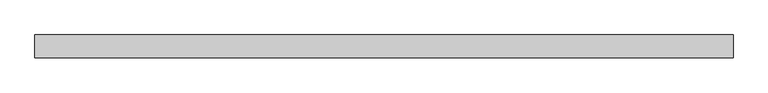
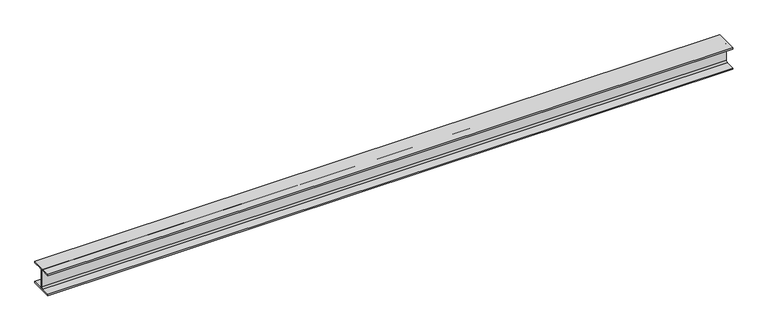
"""IFC4 building model written with IfcOpenShell, lengths in millimetres: beam geometry, 0912_Steel Framing_H-KSD3502 : H_SB_ASB_H-200x200x8x12."""

import ifcopenshell
import ifcopenshell.guid

model = None  # the IFC model being written
_history = None  # IfcOwnerHistory: only IFC2X3 demands one
_inside = {}  # id of a spatial element -> (the spatial element, [elements in it])
_under = {}  # id of a project, library or spatial element -> (it, [spatial elements below it])
_declared = {}  # id of a project -> (the project, [libraries it declares])
_typed = {}  # id of a type object -> (the type object, [elements of that type])
_made_of = {}  # id of a material, layer set ... -> (it, [elements and type objects made of it])


def new_model(schema):
    """Start an empty IFC model of exactly this schema.

    Asked for "IFC4X3", IfcOpenShell would pick the latest addendum, in which some entities
    have other attributes; the version numbers below select the first issue.
    IFC2X3 requires an IfcOwnerHistory on every rooted entity: one is made here for all.
    """
    global model, _history
    if schema == "IFC4X3":
        model = ifcopenshell.file(schema_version=(4, 3, 0, 0))
    else:
        model = ifcopenshell.file(schema=schema)
    _inside.clear()
    _under.clear()
    _declared.clear()
    _typed.clear()
    _made_of.clear()
    _history = None
    if model.schema == "IFC2X3":
        org = make("IfcOrganization", Name="unknown")
        user = make(
            "IfcPersonAndOrganization",
            ThePerson=make("IfcPerson", FamilyName="unknown"),
            TheOrganization=org,
        )
        app = make(
            "IfcApplication",
            ApplicationDeveloper=org,
            Version="unknown",
            ApplicationFullName="unknown",
            ApplicationIdentifier="unknown",
        )
        _history = make(
            "IfcOwnerHistory",
            OwningUser=user,
            OwningApplication=app,
            ChangeAction="ADDED",
            CreationDate=0,
        )
    return model


def make(cls, **values):
    """One entity of the class cls with the attributes given. An attribute that is None is left unset."""
    return model.create_entity(
        cls, **{name: value for name, value in values.items() if value is not None}
    )


def rooted(cls, **values):
    """An entity with a GlobalId (a new one), such as an element, a storey or a relation."""
    return make(cls, GlobalId=ifcopenshell.guid.new(), OwnerHistory=_history, **values)


def si_unit(unit_type, name, prefix=None):
    """IfcSIUnit, for example si_unit("LENGTHUNIT", "METRE", prefix="MILLI")."""
    return make("IfcSIUnit", UnitType=unit_type, Prefix=prefix, Name=name)


def assignment(units):
    """IfcUnitAssignment: the units of a project."""
    return None if units is None else make("IfcUnitAssignment", Units=units)


def point(xyz):
    """IfcCartesianPoint."""
    return None if xyz is None else make("IfcCartesianPoint", Coordinates=xyz)


def direction(xyz):
    """IfcDirection."""
    return None if xyz is None else make("IfcDirection", DirectionRatios=xyz)


def frame(location, z_axis=None, x_axis=None):
    """IfcAxis2Placement3D, a coordinate frame: its origin and axes. An axis left out is left unset."""
    return make(
        "IfcAxis2Placement3D",
        Location=point(location),
        Axis=direction(z_axis),
        RefDirection=direction(x_axis),
    )


def frame_2d(location, x_axis=None):
    """IfcAxis2Placement2D, a coordinate frame in the plane: its origin and x axis."""
    return make(
        "IfcAxis2Placement2D", Location=point(location), RefDirection=direction(x_axis)
    )


def origin():
    """The frame at (0, 0, 0) with its axes left unset."""
    return frame((0.0, 0.0, 0.0))


def place(relative_to, where):
    """IfcLocalPlacement: puts the frame where relative to a parent placement (None: the world)."""
    return make(
        "IfcLocalPlacement", PlacementRelTo=relative_to, RelativePlacement=where
    )


def context(
    kind, dimensions, precision=None, world=None, true_north=None, identifier=None
):
    """IfcGeometricRepresentationContext, for example the 3D "Model" context."""
    return make(
        "IfcGeometricRepresentationContext",
        ContextIdentifier=identifier,
        ContextType=kind,
        CoordinateSpaceDimension=dimensions,
        Precision=precision,
        WorldCoordinateSystem=world,
        TrueNorth=true_north,
    )


def project(units=None, contexts=None):
    """IfcProject with its units and contexts."""
    return rooted(
        "IfcProject",
        Name="project",
        RepresentationContexts=contexts,
        UnitsInContext=assignment(units),
    )


def spatial(cls, under=None, at=None, **own):
    """A site, building, storey or space (cls), placed at a placement, below another one or the project."""
    s = rooted(cls, ObjectPlacement=at, **own)
    if under is not None:
        _under.setdefault(under.id(), (under, []))[1].append(s)
    return s


def polyline(points):
    """IfcPolyline through the points."""
    return make("IfcPolyline", Points=[point(p) for p in points])


def circle_curve(where, radius):
    """IfcCircle in the frame where."""
    return make("IfcCircle", Position=where, Radius=radius)


def trimmed(basis, trim1, trim2, sense, master):
    """IfcTrimmedCurve: the piece of a basis curve between two trims."""
    return make(
        "IfcTrimmedCurve",
        BasisCurve=basis,
        Trim1=trim1,
        Trim2=trim2,
        SenseAgreement=sense,
        MasterRepresentation=master,
    )


def segment(curve, same_sense, transition):
    """IfcCompositeCurveSegment."""
    return make(
        "IfcCompositeCurveSegment",
        Transition=transition,
        SameSense=same_sense,
        ParentCurve=curve,
    )


def composite_curve(segments, self_intersect=None):
    """IfcCompositeCurve: segments joined end to end."""
    return make("IfcCompositeCurve", Segments=segments, SelfIntersect=self_intersect)


def outline(outer, holes=None, kind="AREA"):
    """IfcArbitraryClosedProfileDef: a profile drawn as a closed curve; with holes, ...WithVoids."""
    if holes is None:
        return make("IfcArbitraryClosedProfileDef", ProfileType=kind, OuterCurve=outer)
    return make(
        "IfcArbitraryProfileDefWithVoids",
        ProfileType=kind,
        OuterCurve=outer,
        InnerCurves=holes,
    )


def extrude(swept, where, along, depth):
    """IfcExtrudedAreaSolid: the profile swept, set in the frame where, extruded along a direction by depth."""
    return make(
        "IfcExtrudedAreaSolid",
        SweptArea=swept,
        Position=where,
        ExtrudedDirection=direction(along),
        Depth=depth,
    )


def shape(context_of_items, identifier, shape_type, items):
    """IfcShapeRepresentation: the items that make up one representation, for example the "Body"."""
    return make(
        "IfcShapeRepresentation",
        ContextOfItems=context_of_items,
        RepresentationIdentifier=identifier,
        RepresentationType=shape_type,
        Items=items,
    )


def source(mapping_origin, context_of_items, identifier, shape_type, items):
    """IfcRepresentationMap: a shape defined once, which mapped items show again and again."""
    return make(
        "IfcRepresentationMap",
        MappingOrigin=mapping_origin,
        MappedRepresentation=shape(context_of_items, identifier, shape_type, items),
    )


def transform(
    local_origin,
    x_axis=None,
    y_axis=None,
    z_axis=None,
    scale=None,
    scale2=None,
    scale3=None,
    uniform=True,
):
    """IfcCartesianTransformationOperator3D, or its non-uniform kind. x_axis, y_axis, z_axis: its Axis1, 2, 3."""
    if uniform:
        return make(
            "IfcCartesianTransformationOperator3D",
            Axis1=direction(x_axis),
            Axis2=direction(y_axis),
            LocalOrigin=point(local_origin),
            Scale=scale,
            Axis3=direction(z_axis),
        )
    return make(
        "IfcCartesianTransformationOperator3DnonUniform",
        Axis1=direction(x_axis),
        Axis2=direction(y_axis),
        LocalOrigin=point(local_origin),
        Scale=scale,
        Axis3=direction(z_axis),
        Scale2=scale2,
        Scale3=scale3,
    )


def mapped(mapping_source, mapping_target):
    """IfcMappedItem: shows the shape of a source again, moved by a transform."""
    return make(
        "IfcMappedItem", MappingSource=mapping_source, MappingTarget=mapping_target
    )


def made_of(thing, what):
    """Note that an element or type object is made of a material, layer set ...; save() writes the relation."""
    if what is not None:
        _made_of.setdefault(what.id(), (what, []))[1].append(thing)
    return thing


def element(
    cls,
    number,
    at=None,
    inside=None,
    cuts=None,
    type_object=None,
    material=None,
    context=None,
    identifier="Body",
    shape_type=None,
    held_by="IfcProductDefinitionShape",
    body=None,
    shapes=None,
    **own,
):
    """One element of the class cls, such as IfcWall. Its Tag is "e" and its number.

    at: its placement. inside: the storey or other place that contains it. cuts: it is an
    opening in that element (IfcRelVoidsElement). A single representation is given by context,
    identifier, shape_type and body (its items); several are given by shapes. held_by: the class
    of the entity that holds the representations. save() writes the other relations.
    """
    e = rooted(cls, Tag="e%d" % number, ObjectPlacement=at, **own)
    if body is not None:
        shapes = [shape(context, identifier, shape_type, body)]
    if shapes is not None:
        e.Representation = make(held_by, Representations=shapes)
    if inside is not None:
        _inside.setdefault(inside.id(), (inside, []))[1].append(e)
    if cuts is not None:
        rooted(
            "IfcRelVoidsElement", RelatingBuildingElement=cuts, RelatedOpeningElement=e
        )
    if type_object is not None:
        _typed.setdefault(type_object.id(), (type_object, []))[1].append(e)
    return made_of(e, material)


def aggregate(whole, parts):
    """IfcRelAggregates: a whole, such as a stair, and the parts it consists of."""
    return rooted("IfcRelAggregates", RelatingObject=whole, RelatedObjects=parts)


def save(model, path):
    """Write the relations noted so far, then the file.

    IfcRelAggregates (storeys below a building ...), IfcRelContainedInSpatialStructure (elements
    in a storey), IfcRelDefinesByType, IfcRelAssociatesMaterial and IfcRelDeclares: one each for
    every whole, place, type object, material and project.
    """
    for whole, parts in _under.values():
        aggregate(whole, parts)
    for where, things in _inside.values():
        rooted(
            "IfcRelContainedInSpatialStructure",
            RelatedElements=things,
            RelatingStructure=where,
        )
    for kind, things in _typed.values():
        rooted("IfcRelDefinesByType", RelatedObjects=things, RelatingType=kind)
    for what, things in _made_of.values():
        rooted("IfcRelAssociatesMaterial", RelatedObjects=things, RelatingMaterial=what)
    for by, libraries in _declared.values():
        rooted("IfcRelDeclares", RelatingContext=by, RelatedDefinitions=libraries)
    model.write(path)


def beam_026c0679(model_context):
    return source(origin(), model_context, "Body", "SweptSolid", [
        extrude(outline(composite_curve([segment(polyline([(100.0, -88.0), (100.0, -100.0), (-100.0, -100.0), (-100.0, -88.0), (-17.0, -88.0)]), True, "CONTINUOUS"), segment(trimmed(circle_curve(frame_2d((-17.0, -75.0)), 13.0), [point((-17.0, -88.0))], [point((-4.0, -75.0))], True, "CARTESIAN"), True, "CONTINUOUS"), segment(polyline([(-4.0, -75.0), (-4.0, 75.0)]), True, "CONTINUOUS"), segment(trimmed(circle_curve(frame_2d((-17.0, 75.0)), 13.0), [point((-4.0, 75.0))], [point((-17.0, 88.0))], True, "CARTESIAN"), True, "CONTINUOUS"), segment(polyline([(-17.0, 88.0), (-100.0, 88.0), (-100.0, 100.0), (100.0, 100.0), (100.0, 88.0), (17.0, 88.0)]), True, "CONTINUOUS"), segment(trimmed(circle_curve(frame_2d((17.0, 75.0)), 13.0), [point((17.0, 88.0))], [point((4.0, 75.0))], True, "CARTESIAN"), True, "CONTINUOUS"), segment(polyline([(4.0, 75.0), (4.0, -75.0)]), True, "CONTINUOUS"), segment(trimmed(circle_curve(frame_2d((17.0, -75.0)), 13.0), [point((4.0, -75.0))], [point((17.0, -88.0))], True, "CARTESIAN"), True, "CONTINUOUS"), segment(polyline([(17.0, -88.0), (100.0, -88.0)]), True, "CONTINUOUS")], self_intersect=False)), frame((-3041.4802947, 0.0, 0.0), z_axis=(1.0, 0.0, 0.0), x_axis=(0.0, 1.0, 0.0)), (0.0, 0.0, 1.0), 6052.7309213),
    ])


if __name__ == "__main__":
    model = new_model("IFC4")
    model_context = context("Model", 3, world=origin())
    ifc_project = project(units=[si_unit("LENGTHUNIT", "METRE", prefix="MILLI")], contexts=[model_context])
    site = spatial("IfcSite", under=ifc_project)
    building = spatial("IfcBuilding", under=site)
    placement = place(None, origin())
    beam_shape = beam_026c0679(model_context)
    element("IfcBeam", 1, ObjectType="0912_Steel Framing_H-KSD3502 : H_SB_ASB_H-200x200x8x12", at=placement, inside=building, context=model_context, shape_type="MappedRepresentation", body=[
        mapped(beam_shape, transform((0.0, 0.0, 0.0), x_axis=(1.0, 0.0, 0.0), y_axis=(0.0, 1.0, 0.0), z_axis=(0.0, 0.0, 1.0))),
    ])
    save(model, "model.ifc")

# Revit data of these elements
# Type "0912_Steel Framing_H-KSD3502 : H_SB_ASB_H-200x200x8x12"
#   H_WM Code_1 = "S01AA002-00001 | Main Steel Structure Fabrication Work | Shelter/Building | Medium Steel - Standard (90KG/M>Weight≥30KG/M) | Material: (   )"
#   H_WM Code_2 = "S03AA028-00001 | Main Steel Structure Erection Work | Shelter/Building | Medium Steel (90KG/M>Weight≥30KG/M) | Material: (   )"
#   H_WM Code_3 = "S01AA010-00001 | Main Steel Structure Fabrication Work | Shelter/Building | Steel Painting/Coating | for Non-Fireproofed Steel Surface, Surface Preparation, Primer, Second & Final Coat | Material: (   )"
#   H_Q'ty Cal Type Tag = "SB-Q2"
#   Width = 20.0 cm
#   Web Thickness = 0.8 cm
#   Web Fillet = 1.3 cm
#   Warping Constant = 141000.0 cm⁶
#   W = 0
#   Torsional Moment of Inertia = 26.2485 cm⁴
#   Section Area = 63.53 cm²
#   Plastic Modulus weak axis = 244.0 cm³
#   Plastic Modulus strong axis = 525.0 cm³
#   Perimeter = 1.16 m²/m
#   Nominal Weight = 49.90 kgf/m
#   Moment of Inertia weak axis = 1600.00 cm⁴
#   Moment of Inertia strong axis = 4720.00 cm⁴
#   Height = 20.0 cm
#   Flange Thickness = 1.2 cm
#   Elastic Modulus weak axis = 160.0 cm³
#   Elastic Modulus strong axis = 472.0 cm³
#   Centroid Vertical = 10.0 cm
#   Centroid Horizontal = 10.0 cm
#   Ix = 47200000
#   Length [instance default] = 1.5240 m
#   Zx = 525000
#   b = 0.2000 m
#   h = 0.2000 m
#   r = 0.0130 m
#   s = 0.0080 m
#   t = 0.0120 m
#   A = 0.006353 m²
#   Structural Material [instance default] = Steel, 45-345
#   Assembly Code = ""
# Element 1 (IfcBeam, "0912_Steel Framing_H-KSD3502 : H_SB_ASB_H-200x200x8x12")
#   Structural Material = none
# Materials
#   "Steel, 45-345": class "Metal", colour RGB 189 187 185, transparency 0, Description = "Steel 345 MPa", Cost = 0
